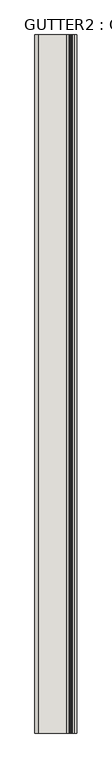
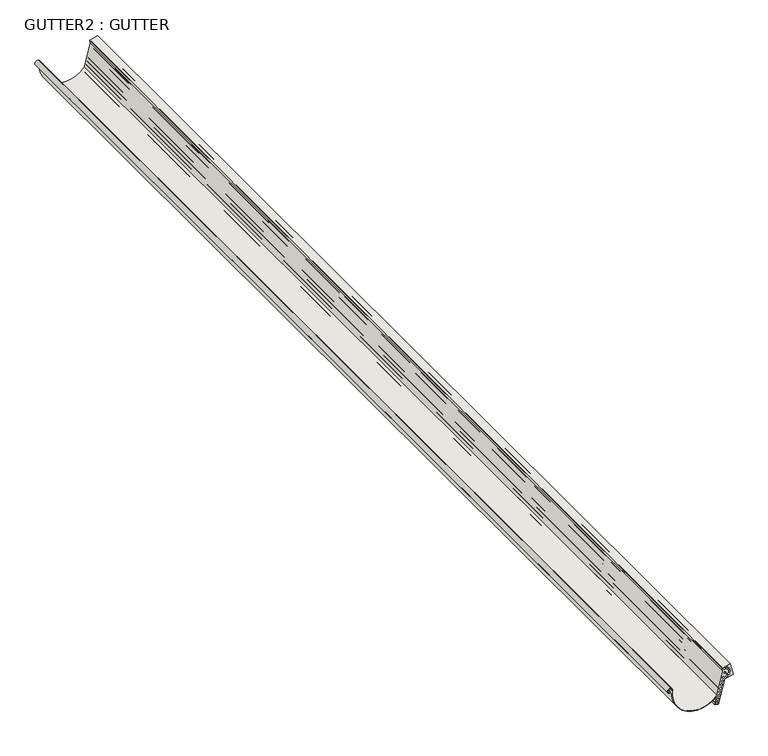
"""IFC4 building model written with IfcOpenShell, lengths in millimetres: wall geometry, GUTTER2 : GUTTER."""

from ifc_helpers import new_model, si_unit, point, frame, frame_2d, origin, place, context, project, spatial, polyline, circle_curve, trimmed, segment, composite_curve, outline, extrude, source, transform, mapped, element, save


def gutter2_gutter_ab6c3562(model_context):
    return source(origin(), model_context, "Body", "SweptSolid", [
        extrude(outline(composite_curve([segment(trimmed(circle_curve(frame_2d((2303.7835273, 17295.7878287)), 67.3753748), [point((2258.1932947, 17345.3960117))], [point((2311.7874564, 17228.8895608))], True, "CARTESIAN"), True, "CONTINUOUS"), segment(trimmed(circle_curve(frame_2d((2314.0265285, 17222.5834829)), 6.6917907), [point((2311.7874564, 17228.8895608))], [point((2307.347541, 17222.9972325))], False, "CARTESIAN"), True, "CONTINUOUS"), segment(polyline([(2307.347541, 17222.9972325), (2313.5940497, 17222.4844423), (2313.5153542, 17221.5258201), (2308.3315579, 17221.9513699)]), True, "CONTINUOUS"), segment(trimmed(circle_curve(frame_2d((2314.0265285, 17222.5834829)), 5.7299439), [point((2308.3315579, 17221.9513699))], [point((2312.0127617, 17227.9479027))], True, "CARTESIAN"), True, "CONTINUOUS"), segment(trimmed(circle_curve(frame_2d((2303.7835273, 17295.7878287)), 68.3372216), [point((2312.0127617, 17227.9479027))], [point((2256.27153, 17344.9059106))], False, "CARTESIAN"), True, "CONTINUOUS"), segment(polyline([(2256.27153, 17344.9059106), (2235.0084979, 17339.4832725), (2232.6495096, 17348.7332432), (2296.8549207, 17365.1073291), (2301.4897637, 17387.5018804), (2333.4799408, 17379.7076452), (2328.4986037, 17359.2625531), (2319.7036418, 17361.0827846), (2258.1932947, 17345.3960117)]), True, "CONTINUOUS")], self_intersect=False), holes=[composite_curve([segment(trimmed(circle_curve(frame_2d((2237.4687582, 17345.6687234)), 2.3644757), [point((2236.8844559, 17347.9598663))], [point((2238.0530605, 17343.3775804))], True, "CARTESIAN"), True, "CONTINUOUS"), segment(trimmed(circle_curve(frame_2d((2237.4687582, 17345.6687234)), 2.3644757), [point((2238.0530605, 17343.3775804))], [point((2236.8844559, 17347.9598663))], True, "CARTESIAN"), True, "CONTINUOUS")], self_intersect=False), composite_curve([segment(trimmed(circle_curve(frame_2d((2246.6983463, 17348.0225136)), 2.3644757), [point((2246.114044, 17350.3136565))], [point((2247.2826487, 17345.7313707))], True, "CARTESIAN"), True, "CONTINUOUS"), segment(trimmed(circle_curve(frame_2d((2246.6983463, 17348.0225136)), 2.3644757), [point((2247.2826487, 17345.7313707))], [point((2246.114044, 17350.3136565))], True, "CARTESIAN"), True, "CONTINUOUS")], self_intersect=False), composite_curve([segment(trimmed(circle_curve(frame_2d((2255.9279344, 17350.3763038)), 2.3644757), [point((2255.3436321, 17352.6674467))], [point((2256.5122368, 17348.0851609))], True, "CARTESIAN"), True, "CONTINUOUS"), segment(trimmed(circle_curve(frame_2d((2255.9279344, 17350.3763038)), 2.3644757), [point((2256.5122368, 17348.0851609))], [point((2255.3436321, 17352.6674467))], True, "CARTESIAN"), True, "CONTINUOUS")], self_intersect=False), composite_curve([segment(trimmed(circle_curve(frame_2d((2265.1575225, 17352.730094)), 2.3644757), [point((2264.5732202, 17355.0212369))], [point((2265.7418249, 17350.4389511))], True, "CARTESIAN"), True, "CONTINUOUS"), segment(trimmed(circle_curve(frame_2d((2265.1575225, 17352.730094)), 2.3644757), [point((2265.7418249, 17350.4389511))], [point((2264.5732202, 17355.0212369))], True, "CARTESIAN"), True, "CONTINUOUS")], self_intersect=False), composite_curve([segment(trimmed(circle_curve(frame_2d((2274.3871107, 17355.0838842)), 2.3644757), [point((2273.8028083, 17357.3750272))], [point((2274.971413, 17352.7927413))], True, "CARTESIAN"), True, "CONTINUOUS"), segment(trimmed(circle_curve(frame_2d((2274.3871107, 17355.0838842)), 2.3644757), [point((2274.971413, 17352.7927413))], [point((2273.8028083, 17357.3750272))], True, "CARTESIAN"), True, "CONTINUOUS")], self_intersect=False), composite_curve([segment(trimmed(circle_curve(frame_2d((2283.6166988, 17357.4376744)), 2.3644757), [point((2283.0323964, 17359.7288174))], [point((2284.2010011, 17355.1465315))], True, "CARTESIAN"), True, "CONTINUOUS"), segment(trimmed(circle_curve(frame_2d((2283.6166988, 17357.4376744)), 2.3644757), [point((2284.2010011, 17355.1465315))], [point((2283.0323964, 17359.7288174))], True, "CARTESIAN"), True, "CONTINUOUS")], self_intersect=False), composite_curve([segment(trimmed(circle_curve(frame_2d((2292.8462869, 17359.7914646)), 2.3644757), [point((2292.2619845, 17362.0826076))], [point((2293.4305892, 17357.5003217))], True, "CARTESIAN"), True, "CONTINUOUS"), segment(trimmed(circle_curve(frame_2d((2292.8462869, 17359.7914646)), 2.3644757), [point((2293.4305892, 17357.5003217))], [point((2292.2619845, 17362.0826076))], True, "CARTESIAN"), True, "CONTINUOUS")], self_intersect=False), composite_curve([segment(trimmed(circle_curve(frame_2d((2302.075875, 17362.1452548)), 2.3644757), [point((2301.4915727, 17364.4363978))], [point((2302.6601773, 17359.8541119))], True, "CARTESIAN"), True, "CONTINUOUS"), segment(trimmed(circle_curve(frame_2d((2302.075875, 17362.1452548)), 2.3644757), [point((2302.6601773, 17359.8541119))], [point((2301.4915727, 17364.4363978))], True, "CARTESIAN"), True, "CONTINUOUS")], self_intersect=False), composite_curve([segment(trimmed(circle_curve(frame_2d((2326.1348247, 17365.0364584)), 2.3644757), [point((2325.5505224, 17367.3276013))], [point((2326.7191271, 17362.7453155))], True, "CARTESIAN"), True, "CONTINUOUS"), segment(trimmed(circle_curve(frame_2d((2326.1348247, 17365.0364584)), 2.3644757), [point((2326.7191271, 17362.7453155))], [point((2325.5505224, 17367.3276013))], True, "CARTESIAN"), True, "CONTINUOUS")], self_intersect=False), composite_curve([segment(trimmed(circle_curve(frame_2d((2314.2554016, 17366.2207206)), 2.3644757), [point((2313.6710993, 17368.5118635))], [point((2314.8397039, 17363.9295777))], True, "CARTESIAN"), True, "CONTINUOUS"), segment(trimmed(circle_curve(frame_2d((2314.2554016, 17366.2207206)), 2.3644757), [point((2314.8397039, 17363.9295777))], [point((2313.6710993, 17368.5118635))], True, "CARTESIAN"), True, "CONTINUOUS")], self_intersect=False), composite_curve([segment(trimmed(circle_curve(frame_2d((2324.9572871, 17371.5115445)), 2.3644757), [point((2323.2476499, 17373.1449108))], [point((2326.6669244, 17369.8781781))], True, "CARTESIAN"), True, "CONTINUOUS"), segment(trimmed(circle_curve(frame_2d((2324.9572871, 17371.5115445)), 2.3644757), [point((2326.6669244, 17369.8781781))], [point((2323.2476499, 17373.1449108))], True, "CARTESIAN"), True, "CONTINUOUS")], self_intersect=False), composite_curve([segment(trimmed(circle_curve(frame_2d((2320.5274058, 17376.378729)), 2.3644757), [point((2318.2119988, 17376.8579325))], [point((2322.8428127, 17375.8995255))], True, "CARTESIAN"), True, "CONTINUOUS"), segment(trimmed(circle_curve(frame_2d((2320.5274058, 17376.378729)), 2.3644757), [point((2322.8428127, 17375.8995255))], [point((2318.2119988, 17376.8579325))], True, "CARTESIAN"), True, "CONTINUOUS")], self_intersect=False), composite_curve([segment(trimmed(circle_curve(frame_2d((2314.1914384, 17378.1588561)), 2.3644757), [point((2311.9739228, 17377.338265))], [point((2316.408954, 17378.9794472))], True, "CARTESIAN"), True, "CONTINUOUS"), segment(trimmed(circle_curve(frame_2d((2314.1914384, 17378.1588561)), 2.3644757), [point((2316.408954, 17378.9794472))], [point((2311.9739228, 17377.338265))], True, "CARTESIAN"), True, "CONTINUOUS")], self_intersect=False), composite_curve([segment(trimmed(circle_curve(frame_2d((2307.8749098, 17376.3109384)), 2.3644757), [point((2306.4291969, 17374.4399334))], [point((2309.3206226, 17378.1819434))], True, "CARTESIAN"), True, "CONTINUOUS"), segment(trimmed(circle_curve(frame_2d((2307.8749098, 17376.3109384)), 2.3644757), [point((2309.3206226, 17378.1819434))], [point((2306.4291969, 17374.4399334))], True, "CARTESIAN"), True, "CONTINUOUS")], self_intersect=False), composite_curve([segment(trimmed(circle_curve(frame_2d((2303.4974369, 17371.3965651)), 2.3644757), [point((2303.2628844, 17369.0437518))], [point((2303.7319893, 17373.7493783))], True, "CARTESIAN"), True, "CONTINUOUS"), segment(trimmed(circle_curve(frame_2d((2303.4974369, 17371.3965651)), 2.3644757), [point((2303.7319893, 17373.7493783))], [point((2303.2628844, 17369.0437518))], True, "CARTESIAN"), True, "CONTINUOUS")], self_intersect=False)]), frame((0.0, -3415.0384634, 0.0), z_axis=(0.0, 1.0, 0.0), x_axis=(0.0, 0.0, 1.0)), (0.0, 0.0, 1.0), 2862.7206389),
    ])


if __name__ == "__main__":
    model = new_model("IFC4")
    model_context = context("Model", 3, world=origin())
    ifc_project = project(units=[si_unit("LENGTHUNIT", "METRE", prefix="MILLI")], contexts=[model_context])
    site = spatial("IfcSite", under=ifc_project)
    building = spatial("IfcBuilding", under=site)
    placement = place(None, origin())
    gutter2_gutter_shape = gutter2_gutter_ab6c3562(model_context)
    element("IfcWall", 1, ObjectType="GUTTER2 : GUTTER", at=placement, inside=building, context=model_context, shape_type="MappedRepresentation", body=[
        mapped(gutter2_gutter_shape, transform((0.0, 0.0, 0.0), x_axis=(1.0, 0.0, 0.0), y_axis=(0.0, 1.0, 0.0), z_axis=(0.0, 0.0, 1.0))),
    ])
    save(model, "model.ifc")

# Revit data of these elements
# Element 1 (IfcWall, "GUTTER2 : GUTTER")
#   Materials on its faces: "HALF ROUND GUTTER - 5\""
# Materials
#   "HALF ROUND GUTTER - 5\"": class "Metal", colour RGB 247 247 247, transparency 0, Description = "Aluminum 6061", Cost = 0
